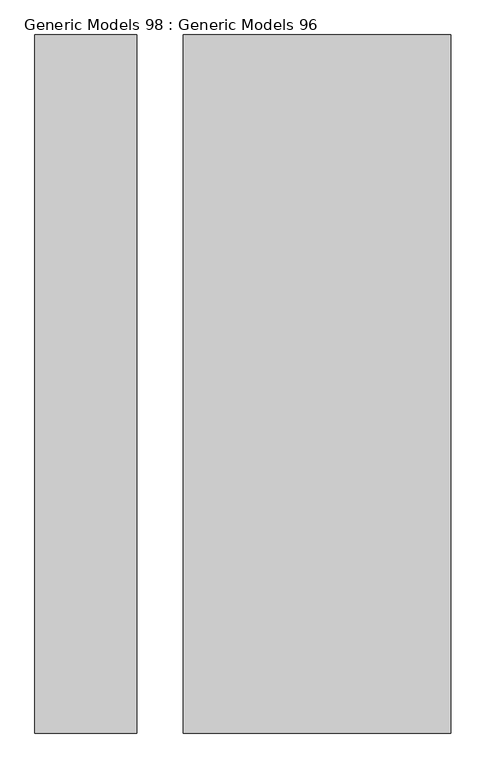
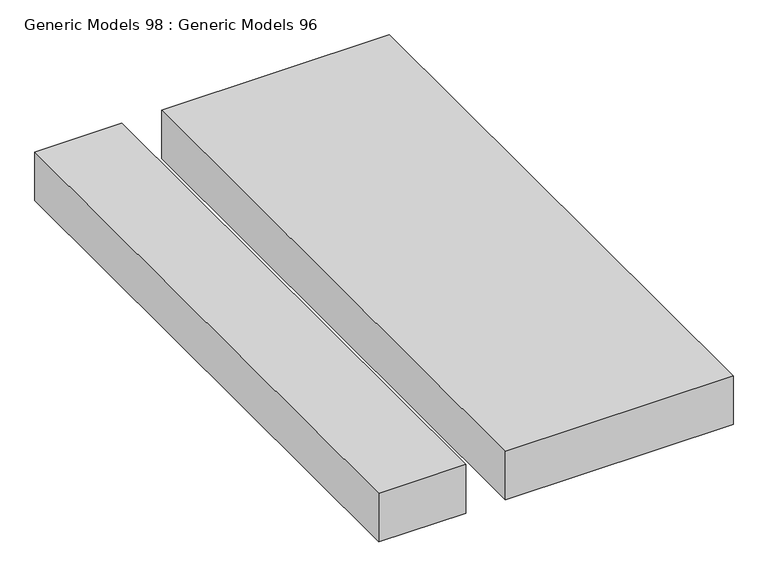
"""IFC4 building model written with IfcOpenShell, lengths in millimetres: proxy geometry, Generic Models 98 : Generic Models 96."""

from ifc_helpers import new_model, si_unit, frame, origin, place, context, project, spatial, polyline, outline, extrude, source, transform, mapped, element, save


def generic_models_98_generic_models_96_57fd75a2(model_context):
    return source(origin(), model_context, "Body", "SweptSolid", [
        extrude(outline(polyline([(20015.0764201, 18191.2264581), (20015.0764201, 21239.2264581), (20460.5616945, 21239.2264581), (20460.5616945, 18191.2264581), (20015.0764201, 18191.2264581)])), frame((0.0, 0.0, 264857.0215033), z_axis=(0.0, 0.0, 1.0), x_axis=(1.0, 0.0, 0.0)), (0.0, 0.0, 1.0), 263.1744143),
        extrude(outline(polyline([(21830.366261, 21239.2264581), (21830.366261, 18191.2264581), (20663.7616945, 18191.2264581), (20663.7616945, 21239.2264581), (21830.366261, 21239.2264581)])), frame((0.0, 0.0, 264857.0215033), z_axis=(0.0, 0.0, 1.0), x_axis=(1.0, 0.0, 0.0)), (0.0, 0.0, 1.0), 263.1744143),
    ])


if __name__ == "__main__":
    model = new_model("IFC4")
    model_context = context("Model", 3, world=origin())
    ifc_project = project(units=[si_unit("LENGTHUNIT", "METRE", prefix="MILLI")], contexts=[model_context])
    site = spatial("IfcSite", under=ifc_project)
    building = spatial("IfcBuilding", under=site)
    placement = place(None, origin())
    generic_models_98_generic_models_96_shape = generic_models_98_generic_models_96_57fd75a2(model_context)
    element("IfcBuildingElementProxy", 1, Name="Generic Models 98 : Generic Models 96", ObjectType="Generic Models 98 : Generic Models 96", at=placement, inside=building, context=model_context, shape_type="MappedRepresentation", body=[
        mapped(generic_models_98_generic_models_96_shape, transform((0.0, 0.0, 0.0), x_axis=(1.0, 0.0, 0.0), y_axis=(0.0, 1.0, 0.0), z_axis=(0.0, 0.0, 1.0))),
    ])
    save(model, "model.ifc")

# Revit data of these elements
# Element 1 (IfcBuildingElementProxy, "Generic Models 98 : Generic Models 96")
#   Materials on its faces: "COMPACTED CRUSHED STONE", "8\" X 3'-6\" DEEP CONCRETE FENCE FOUNDATION (6\" CURB ABOVE GRADE)"
# Materials
#   "COMPACTED CRUSHED STONE": class "Generic", colour RGB 255 255 255, transparency 0, Cost = 0
#   "8\" X 3'-6\" DEEP CONCRETE FENCE FOUNDATION (6\" CURB ABOVE GRADE)": class "Concrete", colour RGB 192 192 192, transparency 0, Description = "Cast-in-place concrete", Cost = 0
